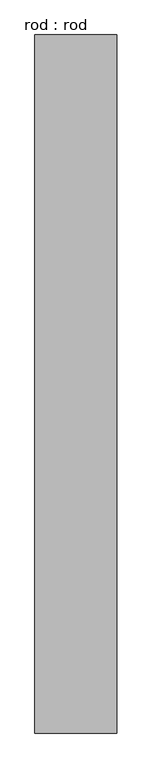
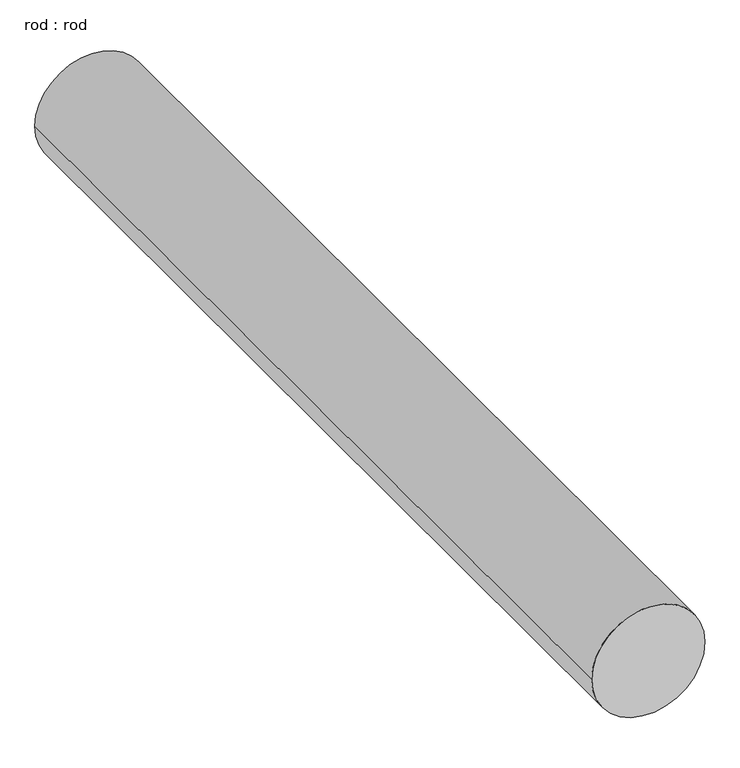
"""IFC4 building model written with IfcOpenShell, lengths in millimetres: proxy geometry, rod : rod."""

from ifc_helpers import new_model, si_unit, point, frame, frame_2d, origin, place, context, project, spatial, circle_curve, trimmed, segment, composite_curve, outline, extrude, source, transform, mapped, element, save


def rod_rod_33799e90(model_context):
    return source(origin(), model_context, "Body", "SweptSolid", [
        extrude(outline(composite_curve([segment(trimmed(circle_curve(frame_2d((0.0108462, 0.0)), 200.0), [point((0.0108462, 200.0))], [point((0.0108462, -200.0))], False, "CARTESIAN"), True, "CONTINUOUS"), segment(trimmed(circle_curve(frame_2d((0.0108462, 0.0)), 200.0), [point((0.0108462, -200.0))], [point((0.0108462, 200.0))], False, "CARTESIAN"), True, "CONTINUOUS")], self_intersect=False)), frame((0.0, 2389.1571868, 0.0), z_axis=(0.0, 1.0, 0.0), x_axis=(0.0, 0.0, 1.0)), (0.0, 0.0, 1.0), 3407.1428571),
    ])


if __name__ == "__main__":
    model = new_model("IFC4")
    model_context = context("Model", 3, world=origin())
    ifc_project = project(units=[si_unit("LENGTHUNIT", "METRE", prefix="MILLI")], contexts=[model_context])
    site = spatial("IfcSite", under=ifc_project)
    building = spatial("IfcBuilding", under=site)
    placement = place(None, origin())
    rod_rod_shape = rod_rod_33799e90(model_context)
    element("IfcBuildingElementProxy", 1, Name="rod : rod", ObjectType="rod : rod", at=placement, inside=building, context=model_context, shape_type="MappedRepresentation", body=[
        mapped(rod_rod_shape, transform((0.0, 0.0, 0.0), x_axis=(1.0, 0.0, 0.0), y_axis=(0.0, 1.0, 0.0), z_axis=(0.0, 0.0, 1.0))),
    ])
    save(model, "model.ifc")

# Revit data of these elements
# Type "rod : rod"
#   Default Elevation = 0
